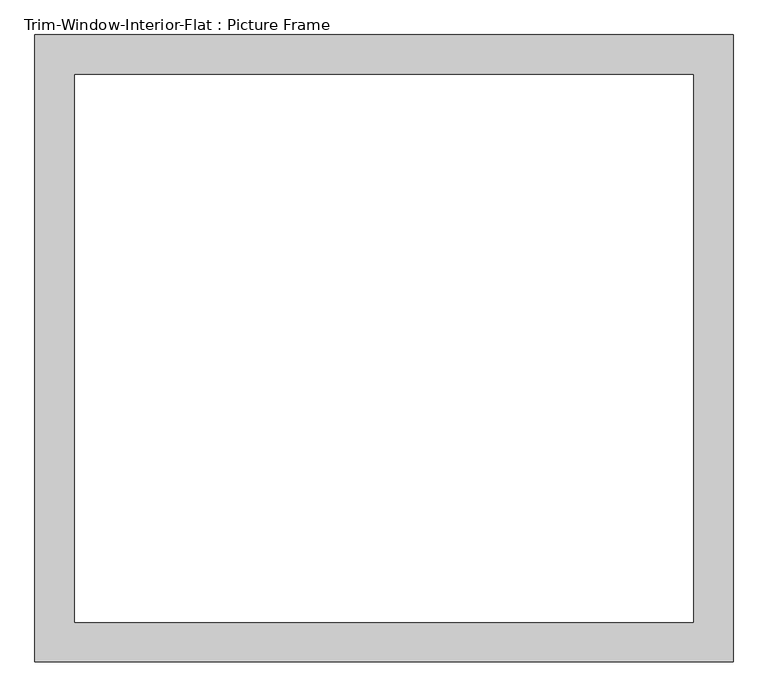
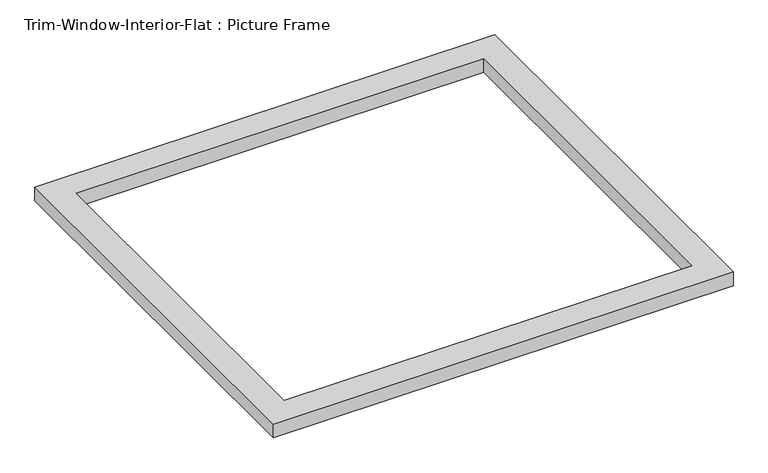
"""IFC4 building model written with IfcOpenShell, lengths in millimetres: proxy geometry, Trim-Window-Interior-Flat : Picture Frame."""

import ifcopenshell
import ifcopenshell.guid

model = None  # the IFC model being written
_history = None  # IfcOwnerHistory: only IFC2X3 demands one
_inside = {}  # id of a spatial element -> (the spatial element, [elements in it])
_under = {}  # id of a project, library or spatial element -> (it, [spatial elements below it])
_declared = {}  # id of a project -> (the project, [libraries it declares])
_typed = {}  # id of a type object -> (the type object, [elements of that type])
_made_of = {}  # id of a material, layer set ... -> (it, [elements and type objects made of it])


def new_model(schema):
    """Start an empty IFC model of exactly this schema.

    Asked for "IFC4X3", IfcOpenShell would pick the latest addendum, in which some entities
    have other attributes; the version numbers below select the first issue.
    IFC2X3 requires an IfcOwnerHistory on every rooted entity: one is made here for all.
    """
    global model, _history
    if schema == "IFC4X3":
        model = ifcopenshell.file(schema_version=(4, 3, 0, 0))
    else:
        model = ifcopenshell.file(schema=schema)
    _inside.clear()
    _under.clear()
    _declared.clear()
    _typed.clear()
    _made_of.clear()
    _history = None
    if model.schema == "IFC2X3":
        org = make("IfcOrganization", Name="unknown")
        user = make(
            "IfcPersonAndOrganization",
            ThePerson=make("IfcPerson", FamilyName="unknown"),
            TheOrganization=org,
        )
        app = make(
            "IfcApplication",
            ApplicationDeveloper=org,
            Version="unknown",
            ApplicationFullName="unknown",
            ApplicationIdentifier="unknown",
        )
        _history = make(
            "IfcOwnerHistory",
            OwningUser=user,
            OwningApplication=app,
            ChangeAction="ADDED",
            CreationDate=0,
        )
    return model


def make(cls, **values):
    """One entity of the class cls with the attributes given. An attribute that is None is left unset."""
    return model.create_entity(
        cls, **{name: value for name, value in values.items() if value is not None}
    )


def rooted(cls, **values):
    """An entity with a GlobalId (a new one), such as an element, a storey or a relation."""
    return make(cls, GlobalId=ifcopenshell.guid.new(), OwnerHistory=_history, **values)


def si_unit(unit_type, name, prefix=None):
    """IfcSIUnit, for example si_unit("LENGTHUNIT", "METRE", prefix="MILLI")."""
    return make("IfcSIUnit", UnitType=unit_type, Prefix=prefix, Name=name)


def assignment(units):
    """IfcUnitAssignment: the units of a project."""
    return None if units is None else make("IfcUnitAssignment", Units=units)


def point(xyz):
    """IfcCartesianPoint."""
    return None if xyz is None else make("IfcCartesianPoint", Coordinates=xyz)


def direction(xyz):
    """IfcDirection."""
    return None if xyz is None else make("IfcDirection", DirectionRatios=xyz)


def frame(location, z_axis=None, x_axis=None):
    """IfcAxis2Placement3D, a coordinate frame: its origin and axes. An axis left out is left unset."""
    return make(
        "IfcAxis2Placement3D",
        Location=point(location),
        Axis=direction(z_axis),
        RefDirection=direction(x_axis),
    )


def origin():
    """The frame at (0, 0, 0) with its axes left unset."""
    return frame((0.0, 0.0, 0.0))


def origin_with_axes():
    """The frame at (0, 0, 0) with the z axis (0, 0, 1) and the x axis (1, 0, 0) written out."""
    return frame((0.0, 0.0, 0.0), z_axis=(0.0, 0.0, 1.0), x_axis=(1.0, 0.0, 0.0))


def place(relative_to, where):
    """IfcLocalPlacement: puts the frame where relative to a parent placement (None: the world)."""
    return make(
        "IfcLocalPlacement", PlacementRelTo=relative_to, RelativePlacement=where
    )


def context(
    kind, dimensions, precision=None, world=None, true_north=None, identifier=None
):
    """IfcGeometricRepresentationContext, for example the 3D "Model" context."""
    return make(
        "IfcGeometricRepresentationContext",
        ContextIdentifier=identifier,
        ContextType=kind,
        CoordinateSpaceDimension=dimensions,
        Precision=precision,
        WorldCoordinateSystem=world,
        TrueNorth=true_north,
    )


def project(units=None, contexts=None):
    """IfcProject with its units and contexts."""
    return rooted(
        "IfcProject",
        Name="project",
        RepresentationContexts=contexts,
        UnitsInContext=assignment(units),
    )


def spatial(cls, under=None, at=None, **own):
    """A site, building, storey or space (cls), placed at a placement, below another one or the project."""
    s = rooted(cls, ObjectPlacement=at, **own)
    if under is not None:
        _under.setdefault(under.id(), (under, []))[1].append(s)
    return s


def polyline(points):
    """IfcPolyline through the points."""
    return make("IfcPolyline", Points=[point(p) for p in points])


def outline(outer, holes=None, kind="AREA"):
    """IfcArbitraryClosedProfileDef: a profile drawn as a closed curve; with holes, ...WithVoids."""
    if holes is None:
        return make("IfcArbitraryClosedProfileDef", ProfileType=kind, OuterCurve=outer)
    return make(
        "IfcArbitraryProfileDefWithVoids",
        ProfileType=kind,
        OuterCurve=outer,
        InnerCurves=holes,
    )


def extrude(swept, where, along, depth):
    """IfcExtrudedAreaSolid: the profile swept, set in the frame where, extruded along a direction by depth."""
    return make(
        "IfcExtrudedAreaSolid",
        SweptArea=swept,
        Position=where,
        ExtrudedDirection=direction(along),
        Depth=depth,
    )


def shape(context_of_items, identifier, shape_type, items):
    """IfcShapeRepresentation: the items that make up one representation, for example the "Body"."""
    return make(
        "IfcShapeRepresentation",
        ContextOfItems=context_of_items,
        RepresentationIdentifier=identifier,
        RepresentationType=shape_type,
        Items=items,
    )


def source(mapping_origin, context_of_items, identifier, shape_type, items):
    """IfcRepresentationMap: a shape defined once, which mapped items show again and again."""
    return make(
        "IfcRepresentationMap",
        MappingOrigin=mapping_origin,
        MappedRepresentation=shape(context_of_items, identifier, shape_type, items),
    )


def transform(
    local_origin,
    x_axis=None,
    y_axis=None,
    z_axis=None,
    scale=None,
    scale2=None,
    scale3=None,
    uniform=True,
):
    """IfcCartesianTransformationOperator3D, or its non-uniform kind. x_axis, y_axis, z_axis: its Axis1, 2, 3."""
    if uniform:
        return make(
            "IfcCartesianTransformationOperator3D",
            Axis1=direction(x_axis),
            Axis2=direction(y_axis),
            LocalOrigin=point(local_origin),
            Scale=scale,
            Axis3=direction(z_axis),
        )
    return make(
        "IfcCartesianTransformationOperator3DnonUniform",
        Axis1=direction(x_axis),
        Axis2=direction(y_axis),
        LocalOrigin=point(local_origin),
        Scale=scale,
        Axis3=direction(z_axis),
        Scale2=scale2,
        Scale3=scale3,
    )


def mapped(mapping_source, mapping_target):
    """IfcMappedItem: shows the shape of a source again, moved by a transform."""
    return make(
        "IfcMappedItem", MappingSource=mapping_source, MappingTarget=mapping_target
    )


def made_of(thing, what):
    """Note that an element or type object is made of a material, layer set ...; save() writes the relation."""
    if what is not None:
        _made_of.setdefault(what.id(), (what, []))[1].append(thing)
    return thing


def element(
    cls,
    number,
    at=None,
    inside=None,
    cuts=None,
    type_object=None,
    material=None,
    context=None,
    identifier="Body",
    shape_type=None,
    held_by="IfcProductDefinitionShape",
    body=None,
    shapes=None,
    **own,
):
    """One element of the class cls, such as IfcWall. Its Tag is "e" and its number.

    at: its placement. inside: the storey or other place that contains it. cuts: it is an
    opening in that element (IfcRelVoidsElement). A single representation is given by context,
    identifier, shape_type and body (its items); several are given by shapes. held_by: the class
    of the entity that holds the representations. save() writes the other relations.
    """
    e = rooted(cls, Tag="e%d" % number, ObjectPlacement=at, **own)
    if body is not None:
        shapes = [shape(context, identifier, shape_type, body)]
    if shapes is not None:
        e.Representation = make(held_by, Representations=shapes)
    if inside is not None:
        _inside.setdefault(inside.id(), (inside, []))[1].append(e)
    if cuts is not None:
        rooted(
            "IfcRelVoidsElement", RelatingBuildingElement=cuts, RelatedOpeningElement=e
        )
    if type_object is not None:
        _typed.setdefault(type_object.id(), (type_object, []))[1].append(e)
    return made_of(e, material)


def aggregate(whole, parts):
    """IfcRelAggregates: a whole, such as a stair, and the parts it consists of."""
    return rooted("IfcRelAggregates", RelatingObject=whole, RelatedObjects=parts)


def save(model, path):
    """Write the relations noted so far, then the file.

    IfcRelAggregates (storeys below a building ...), IfcRelContainedInSpatialStructure (elements
    in a storey), IfcRelDefinesByType, IfcRelAssociatesMaterial and IfcRelDeclares: one each for
    every whole, place, type object, material and project.
    """
    for whole, parts in _under.values():
        aggregate(whole, parts)
    for where, things in _inside.values():
        rooted(
            "IfcRelContainedInSpatialStructure",
            RelatedElements=things,
            RelatingStructure=where,
        )
    for kind, things in _typed.values():
        rooted("IfcRelDefinesByType", RelatedObjects=things, RelatingType=kind)
    for what, things in _made_of.values():
        rooted("IfcRelAssociatesMaterial", RelatedObjects=things, RelatingMaterial=what)
    for by, libraries in _declared.values():
        rooted("IfcRelDeclares", RelatingContext=by, RelatedDefinitions=libraries)
    model.write(path)


def trim_window_interior_flat_picture_frame_c9ba522f(model_context):
    return source(origin(), model_context, "Body", "SweptSolid", [
        extrude(outline(polyline([(501.65, 44.45), (501.65, -857.25), (-501.65, -857.25), (-501.65, 44.45), (501.65, 44.45)]), holes=[polyline([(444.5, -12.7), (-444.5, -12.7), (-444.5, -800.1), (444.5, -800.1), (444.5, -12.7)])]), origin_with_axes(), (0.0, 0.0, 1.0), 31.75),
    ])


if __name__ == "__main__":
    model = new_model("IFC4")
    model_context = context("Model", 3, world=origin())
    ifc_project = project(units=[si_unit("LENGTHUNIT", "METRE", prefix="MILLI")], contexts=[model_context])
    site = spatial("IfcSite", under=ifc_project)
    building = spatial("IfcBuilding", under=site)
    placement = place(None, origin())
    trim_window_interior_flat_picture_frame_shape = trim_window_interior_flat_picture_frame_c9ba522f(model_context)
    element("IfcBuildingElementProxy", 1, Name="Trim-Window-Interior-Flat : Picture Frame", ObjectType="Trim-Window-Interior-Flat : Picture Frame", at=placement, inside=building, context=model_context, shape_type="MappedRepresentation", body=[
        mapped(trim_window_interior_flat_picture_frame_shape, transform((0.0, 0.0, 0.0), x_axis=(1.0, 0.0, 0.0), y_axis=(0.0, 1.0, 0.0), z_axis=(0.0, 0.0, 1.0))),
    ])
    save(model, "model.ifc")

# Revit data of these elements
# Type "Trim-Window-Interior-Flat : Picture Frame"
#   Trim Thickness_Picture Frame = 0' - 1 1/4"
#   Trim Width = 0' - 2 1/4"
#   Trim Thickness_with Sill = 0' - 0 3/4"
#   Sill Thickness = 0' - 1 1/4"
#   Opening Width [instance default] = 2' - 0"
#   Opening Height [instance default] = 3' - 0"
#   Default Elevation = 4' - 0"
#   Sill = no
#   Picture Frame = yes
#   Trim Material [instance default] = none
# Element 1 (IfcBuildingElementProxy, "Trim-Window-Interior-Flat : Picture Frame")
#   Opening Width = 3' - 0"
#   Opening Height = 2' - 8"
#   Trim Material = Wood - Stained
#   Materials on its faces: "Wood - Stained"
# Materials
#   "Wood - Stained": class "Wood", colour RGB 224 178 126, transparency 0, Cost = 0
